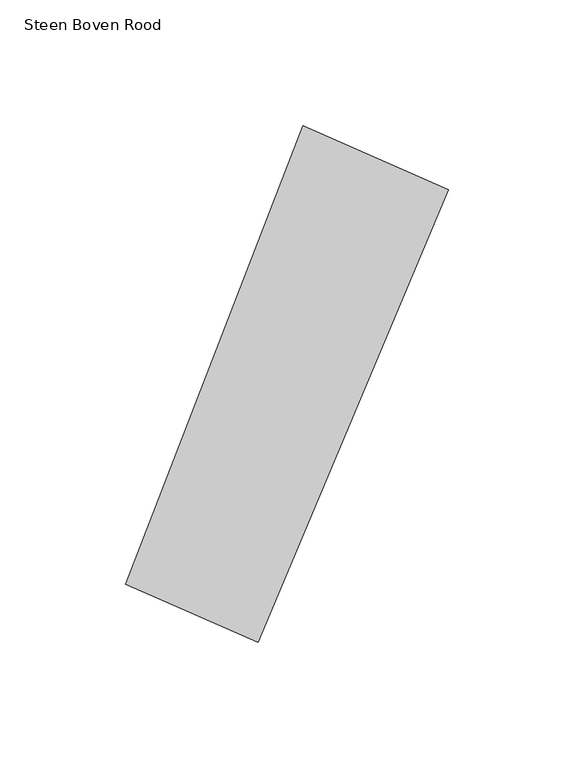
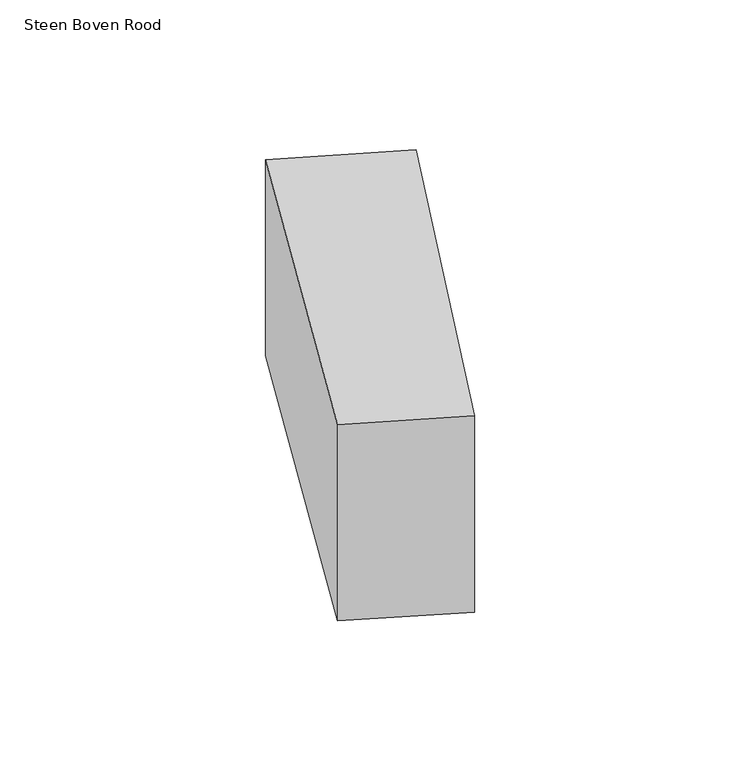
"""IFC4 building model written with IfcOpenShell, lengths in millimetres: proxy geometry, 00_GMA_steen_versie_4 : Steen Boven Rood."""

from ifc_helpers import new_model, si_unit, origin, origin_with_axes, place, context, project, spatial, polyline, outline, extrude, source, transform, mapped, element, save


def steen_boven_rood_be424927(model_context):
    return source(origin(), model_context, "Body", "SweptSolid", [
        extrude(outline(polyline([(139.7467848, 162.7904886), (64.1376003, -16.9779887), (11.5777472, 6.0339625), (81.9668719, 188.092265), (139.7467848, 162.7904886)])), origin_with_axes(), (0.0, 0.0, 1.0), 100.0),
    ])


if __name__ == "__main__":
    model = new_model("IFC4")
    model_context = context("Model", 3, world=origin())
    ifc_project = project(units=[si_unit("LENGTHUNIT", "METRE", prefix="MILLI")], contexts=[model_context])
    site = spatial("IfcSite", under=ifc_project)
    building = spatial("IfcBuilding", under=site)
    placement = place(None, origin())
    steen_boven_rood_shape = steen_boven_rood_be424927(model_context)
    element("IfcBuildingElementProxy", 1, Name="00_GMA_steen_versie_4 : Steen Boven Rood", ObjectType="00_GMA_steen_versie_4 : Steen Boven Rood", at=placement, inside=building, context=model_context, shape_type="MappedRepresentation", body=[
        mapped(steen_boven_rood_shape, transform((0.0, 0.0, 0.0), x_axis=(1.0, 0.0, 0.0), y_axis=(0.0, 1.0, 0.0), z_axis=(0.0, 0.0, 1.0))),
    ])
    save(model, "model.ifc")

# Revit data of these elements
# Type "00_GMA_steen_versie_4 : Steen Boven Rood"
#   StootVoegHalfBoven [instance default] = 5 mm
#   StootVoegHalf [instance default] = 5 mm
#   StootVoegBreedteOnder = 10 mm
#   StootVoegBreedteBoven = 10 mm
#   Steendikte = 100 mm
#   LintVoegOnderHalf = 5 mm
#   LintVoegOnder = 10 mm
#   LintVoegBovenHalf = 0 mm
#   LintVoegBoven = 0 mm
#   materiaal = 21_steen_rood
#   MateriaalVoeg = none
#   Default Elevation = 0
# Element 1 (IfcBuildingElementProxy, "00_GMA_steen_versie_4 : Steen Boven Rood")
#   Materials on its faces: "21_steen_rood"
# Materials
#   "21_steen_rood": class "Unassigned", colour RGB 213 111 43, transparency 0, Cost = 0
